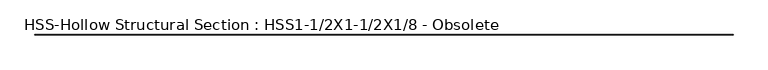
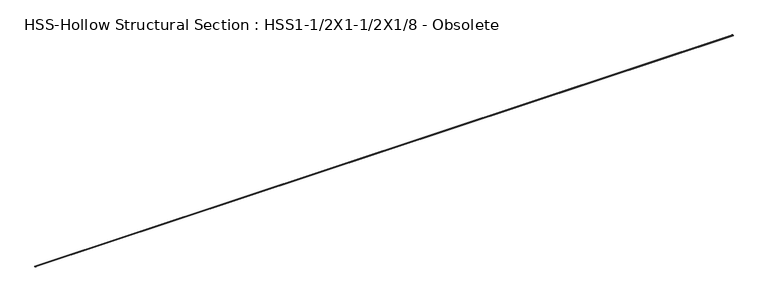
"""IFC4 building model written with IfcOpenShell, lengths in millimetres: beam geometry, HSS-Hollow Structural Section : HSS1-1/2X1-1/2X1/8 - Obsolete."""

from ifc_helpers import new_model, si_unit, point, frame, frame_2d, origin, place, context, project, spatial, polyline, circle_curve, trimmed, segment, composite_curve, outline, extrude, source, transform, mapped, element, save


def hss_hollow_structural_section_hss1_1_2x1_1_2x1_8_obsolete_d4f5de55(model_context):
    return source(origin(), model_context, "Body", "SweptSolid", [
        extrude(outline(composite_curve([segment(polyline([(19.05, 13.1572), (19.05, -13.1572)]), True, "CONTINUOUS"), segment(trimmed(circle_curve(frame_2d((13.1572, -13.1572)), 5.8928), [point((19.05, -13.1572))], [point((13.1572, -19.05))], False, "CARTESIAN"), True, "CONTINUOUS"), segment(polyline([(13.1572, -19.05), (-13.1572, -19.05)]), True, "CONTINUOUS"), segment(trimmed(circle_curve(frame_2d((-13.1572, -13.1572)), 5.8928), [point((-13.1572, -19.05))], [point((-19.05, -13.1572))], False, "CARTESIAN"), True, "CONTINUOUS"), segment(polyline([(-19.05, -13.1572), (-19.05, 13.1572)]), True, "CONTINUOUS"), segment(trimmed(circle_curve(frame_2d((-13.1572, 13.1572)), 5.8928), [point((-19.05, 13.1572))], [point((-13.1572, 19.05))], False, "CARTESIAN"), True, "CONTINUOUS"), segment(polyline([(-13.1572, 19.05), (13.1572, 19.05)]), True, "CONTINUOUS"), segment(trimmed(circle_curve(frame_2d((13.1572, 13.1572)), 5.8928), [point((13.1572, 19.05))], [point((19.05, 13.1572))], False, "CARTESIAN"), True, "CONTINUOUS")], self_intersect=False), holes=[composite_curve([segment(trimmed(circle_curve(frame_2d((-13.1572, 13.1572)), 2.9464), [point((-13.1572, 16.1036))], [point((-16.1036, 13.1572))], True, "CARTESIAN"), True, "CONTINUOUS"), segment(polyline([(-16.1036, 13.1572), (-16.1036, -13.1572)]), True, "CONTINUOUS"), segment(trimmed(circle_curve(frame_2d((-13.1572, -13.1572)), 2.9464), [point((-16.1036, -13.1572))], [point((-13.1572, -16.1036))], True, "CARTESIAN"), True, "CONTINUOUS"), segment(polyline([(-13.1572, -16.1036), (13.1572, -16.1036)]), True, "CONTINUOUS"), segment(trimmed(circle_curve(frame_2d((13.1572, -13.1572)), 2.9464), [point((13.1572, -16.1036))], [point((16.1036, -13.1572))], True, "CARTESIAN"), True, "CONTINUOUS"), segment(polyline([(16.1036, -13.1572), (16.1036, 13.1572)]), True, "CONTINUOUS"), segment(trimmed(circle_curve(frame_2d((13.1572, 13.1572)), 2.9464), [point((16.1036, 13.1572))], [point((13.1572, 16.1036))], True, "CARTESIAN"), True, "CONTINUOUS"), segment(polyline([(13.1572, 16.1036), (-13.1572, 16.1036)]), True, "CONTINUOUS")], self_intersect=False)]), frame((-24507.825, 0.0, 0.0), z_axis=(1.0, 0.0, 0.0), x_axis=(0.0, 1.0, 0.0)), (0.0, 0.0, 1.0), 49015.65),
    ])


if __name__ == "__main__":
    model = new_model("IFC4")
    model_context = context("Model", 3, world=origin())
    ifc_project = project(units=[si_unit("LENGTHUNIT", "METRE", prefix="MILLI")], contexts=[model_context])
    site = spatial("IfcSite", under=ifc_project)
    building = spatial("IfcBuilding", under=site)
    placement = place(None, origin())
    hss_hollow_structural_section_hss1_1_2x1_1_2x1_8_obsolete_shape = hss_hollow_structural_section_hss1_1_2x1_1_2x1_8_obsolete_d4f5de55(model_context)
    element("IfcBeam", 1, ObjectType="HSS-Hollow Structural Section : HSS1-1/2X1-1/2X1/8 - Obsolete", at=placement, inside=building, context=model_context, shape_type="MappedRepresentation", body=[
        mapped(hss_hollow_structural_section_hss1_1_2x1_1_2x1_8_obsolete_shape, transform((0.0, 0.0, 0.0), x_axis=(1.0, 0.0, 0.0), y_axis=(0.0, 1.0, 0.0), z_axis=(0.0, 0.0, 1.0))),
    ])
    save(model, "model.ifc")

# Revit data of these elements
# Type "HSS-Hollow Structural Section : HSS1-1/2X1-1/2X1/8 - Obsolete"
#   Assembly Code = "B10"
#   Shape = "Square"
#   W = 2.19
#   Ht = 0' - 1 1/2"
#   Length [instance default] = 5' - 0"
#   b = 0' - 1 1/2"
#   kr = 0' - 0.232"
#   t = 0' - 0.116"
#   A = 0.00423611 SF
#   Structural Material [instance default] = 1 1/2" X 1 1/2" x 1/8" ALUM. TUBE
# Element 1 (IfcBeam, "HSS-Hollow Structural Section : HSS1-1/2X1-1/2X1/8 - Obsolete")
#   Materials on its faces: "1 1/2\" X 1 1/2\" x 1/8\" ALUM. TUBE"
# Materials
#   "1 1/2\" X 1 1/2\" x 1/8\" ALUM. TUBE": class "Metal", colour RGB 199 199 199, transparency 0, Description = "Carbon steel", Cost = 0
